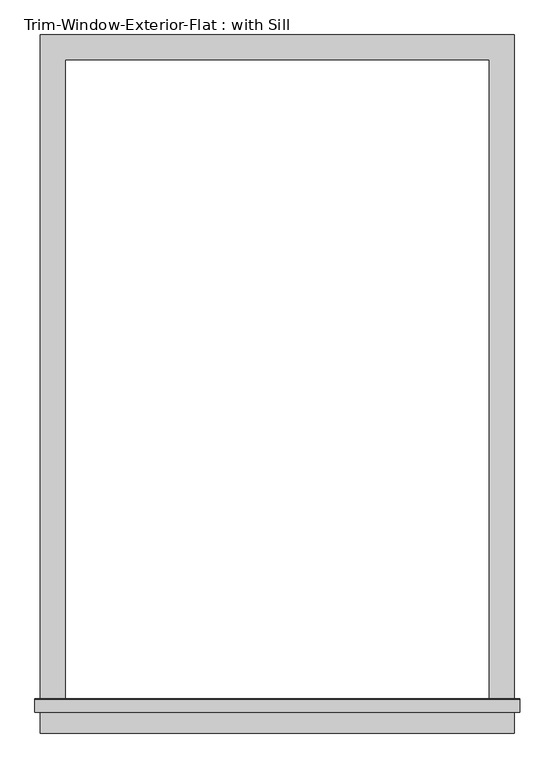
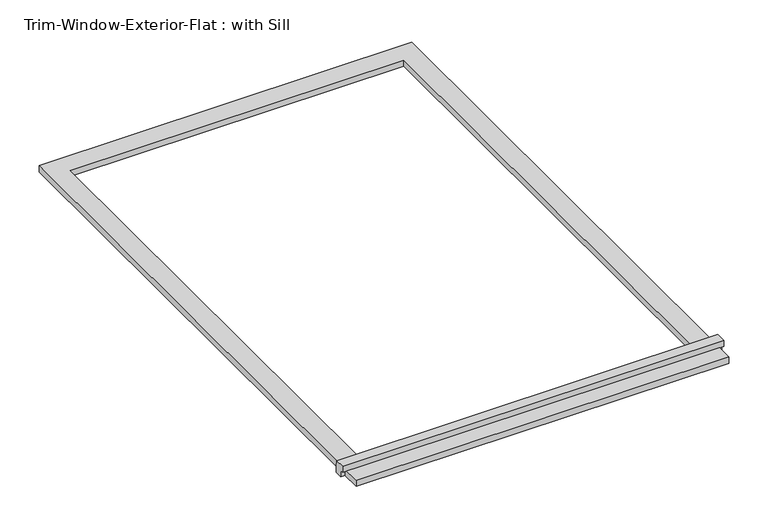
"""IFC4 building model written with IfcOpenShell, lengths in millimetres: proxy geometry, Trim-Window-Exterior-Flat : with Sill."""

import ifcopenshell
import ifcopenshell.guid

model = None  # the IFC model being written
_history = None  # IfcOwnerHistory: only IFC2X3 demands one
_inside = {}  # id of a spatial element -> (the spatial element, [elements in it])
_under = {}  # id of a project, library or spatial element -> (it, [spatial elements below it])
_declared = {}  # id of a project -> (the project, [libraries it declares])
_typed = {}  # id of a type object -> (the type object, [elements of that type])
_made_of = {}  # id of a material, layer set ... -> (it, [elements and type objects made of it])


def new_model(schema):
    """Start an empty IFC model of exactly this schema.

    Asked for "IFC4X3", IfcOpenShell would pick the latest addendum, in which some entities
    have other attributes; the version numbers below select the first issue.
    IFC2X3 requires an IfcOwnerHistory on every rooted entity: one is made here for all.
    """
    global model, _history
    if schema == "IFC4X3":
        model = ifcopenshell.file(schema_version=(4, 3, 0, 0))
    else:
        model = ifcopenshell.file(schema=schema)
    _inside.clear()
    _under.clear()
    _declared.clear()
    _typed.clear()
    _made_of.clear()
    _history = None
    if model.schema == "IFC2X3":
        org = make("IfcOrganization", Name="unknown")
        user = make(
            "IfcPersonAndOrganization",
            ThePerson=make("IfcPerson", FamilyName="unknown"),
            TheOrganization=org,
        )
        app = make(
            "IfcApplication",
            ApplicationDeveloper=org,
            Version="unknown",
            ApplicationFullName="unknown",
            ApplicationIdentifier="unknown",
        )
        _history = make(
            "IfcOwnerHistory",
            OwningUser=user,
            OwningApplication=app,
            ChangeAction="ADDED",
            CreationDate=0,
        )
    return model


def make(cls, **values):
    """One entity of the class cls with the attributes given. An attribute that is None is left unset."""
    return model.create_entity(
        cls, **{name: value for name, value in values.items() if value is not None}
    )


def rooted(cls, **values):
    """An entity with a GlobalId (a new one), such as an element, a storey or a relation."""
    return make(cls, GlobalId=ifcopenshell.guid.new(), OwnerHistory=_history, **values)


def si_unit(unit_type, name, prefix=None):
    """IfcSIUnit, for example si_unit("LENGTHUNIT", "METRE", prefix="MILLI")."""
    return make("IfcSIUnit", UnitType=unit_type, Prefix=prefix, Name=name)


def assignment(units):
    """IfcUnitAssignment: the units of a project."""
    return None if units is None else make("IfcUnitAssignment", Units=units)


def point(xyz):
    """IfcCartesianPoint."""
    return None if xyz is None else make("IfcCartesianPoint", Coordinates=xyz)


def direction(xyz):
    """IfcDirection."""
    return None if xyz is None else make("IfcDirection", DirectionRatios=xyz)


def frame(location, z_axis=None, x_axis=None):
    """IfcAxis2Placement3D, a coordinate frame: its origin and axes. An axis left out is left unset."""
    return make(
        "IfcAxis2Placement3D",
        Location=point(location),
        Axis=direction(z_axis),
        RefDirection=direction(x_axis),
    )


def origin():
    """The frame at (0, 0, 0) with its axes left unset."""
    return frame((0.0, 0.0, 0.0))


def origin_with_axes():
    """The frame at (0, 0, 0) with the z axis (0, 0, 1) and the x axis (1, 0, 0) written out."""
    return frame((0.0, 0.0, 0.0), z_axis=(0.0, 0.0, 1.0), x_axis=(1.0, 0.0, 0.0))


def place(relative_to, where):
    """IfcLocalPlacement: puts the frame where relative to a parent placement (None: the world)."""
    return make(
        "IfcLocalPlacement", PlacementRelTo=relative_to, RelativePlacement=where
    )


def context(
    kind, dimensions, precision=None, world=None, true_north=None, identifier=None
):
    """IfcGeometricRepresentationContext, for example the 3D "Model" context."""
    return make(
        "IfcGeometricRepresentationContext",
        ContextIdentifier=identifier,
        ContextType=kind,
        CoordinateSpaceDimension=dimensions,
        Precision=precision,
        WorldCoordinateSystem=world,
        TrueNorth=true_north,
    )


def project(units=None, contexts=None):
    """IfcProject with its units and contexts."""
    return rooted(
        "IfcProject",
        Name="project",
        RepresentationContexts=contexts,
        UnitsInContext=assignment(units),
    )


def spatial(cls, under=None, at=None, **own):
    """A site, building, storey or space (cls), placed at a placement, below another one or the project."""
    s = rooted(cls, ObjectPlacement=at, **own)
    if under is not None:
        _under.setdefault(under.id(), (under, []))[1].append(s)
    return s


def polyline(points):
    """IfcPolyline through the points."""
    return make("IfcPolyline", Points=[point(p) for p in points])


def outline(outer, holes=None, kind="AREA"):
    """IfcArbitraryClosedProfileDef: a profile drawn as a closed curve; with holes, ...WithVoids."""
    if holes is None:
        return make("IfcArbitraryClosedProfileDef", ProfileType=kind, OuterCurve=outer)
    return make(
        "IfcArbitraryProfileDefWithVoids",
        ProfileType=kind,
        OuterCurve=outer,
        InnerCurves=holes,
    )


def extrude(swept, where, along, depth):
    """IfcExtrudedAreaSolid: the profile swept, set in the frame where, extruded along a direction by depth."""
    return make(
        "IfcExtrudedAreaSolid",
        SweptArea=swept,
        Position=where,
        ExtrudedDirection=direction(along),
        Depth=depth,
    )


def shape(context_of_items, identifier, shape_type, items):
    """IfcShapeRepresentation: the items that make up one representation, for example the "Body"."""
    return make(
        "IfcShapeRepresentation",
        ContextOfItems=context_of_items,
        RepresentationIdentifier=identifier,
        RepresentationType=shape_type,
        Items=items,
    )


def source(mapping_origin, context_of_items, identifier, shape_type, items):
    """IfcRepresentationMap: a shape defined once, which mapped items show again and again."""
    return make(
        "IfcRepresentationMap",
        MappingOrigin=mapping_origin,
        MappedRepresentation=shape(context_of_items, identifier, shape_type, items),
    )


def transform(
    local_origin,
    x_axis=None,
    y_axis=None,
    z_axis=None,
    scale=None,
    scale2=None,
    scale3=None,
    uniform=True,
):
    """IfcCartesianTransformationOperator3D, or its non-uniform kind. x_axis, y_axis, z_axis: its Axis1, 2, 3."""
    if uniform:
        return make(
            "IfcCartesianTransformationOperator3D",
            Axis1=direction(x_axis),
            Axis2=direction(y_axis),
            LocalOrigin=point(local_origin),
            Scale=scale,
            Axis3=direction(z_axis),
        )
    return make(
        "IfcCartesianTransformationOperator3DnonUniform",
        Axis1=direction(x_axis),
        Axis2=direction(y_axis),
        LocalOrigin=point(local_origin),
        Scale=scale,
        Axis3=direction(z_axis),
        Scale2=scale2,
        Scale3=scale3,
    )


def mapped(mapping_source, mapping_target):
    """IfcMappedItem: shows the shape of a source again, moved by a transform."""
    return make(
        "IfcMappedItem", MappingSource=mapping_source, MappingTarget=mapping_target
    )


def made_of(thing, what):
    """Note that an element or type object is made of a material, layer set ...; save() writes the relation."""
    if what is not None:
        _made_of.setdefault(what.id(), (what, []))[1].append(thing)
    return thing


def element(
    cls,
    number,
    at=None,
    inside=None,
    cuts=None,
    type_object=None,
    material=None,
    context=None,
    identifier="Body",
    shape_type=None,
    held_by="IfcProductDefinitionShape",
    body=None,
    shapes=None,
    **own,
):
    """One element of the class cls, such as IfcWall. Its Tag is "e" and its number.

    at: its placement. inside: the storey or other place that contains it. cuts: it is an
    opening in that element (IfcRelVoidsElement). A single representation is given by context,
    identifier, shape_type and body (its items); several are given by shapes. held_by: the class
    of the entity that holds the representations. save() writes the other relations.
    """
    e = rooted(cls, Tag="e%d" % number, ObjectPlacement=at, **own)
    if body is not None:
        shapes = [shape(context, identifier, shape_type, body)]
    if shapes is not None:
        e.Representation = make(held_by, Representations=shapes)
    if inside is not None:
        _inside.setdefault(inside.id(), (inside, []))[1].append(e)
    if cuts is not None:
        rooted(
            "IfcRelVoidsElement", RelatingBuildingElement=cuts, RelatedOpeningElement=e
        )
    if type_object is not None:
        _typed.setdefault(type_object.id(), (type_object, []))[1].append(e)
    return made_of(e, material)


def aggregate(whole, parts):
    """IfcRelAggregates: a whole, such as a stair, and the parts it consists of."""
    return rooted("IfcRelAggregates", RelatingObject=whole, RelatedObjects=parts)


def save(model, path):
    """Write the relations noted so far, then the file.

    IfcRelAggregates (storeys below a building ...), IfcRelContainedInSpatialStructure (elements
    in a storey), IfcRelDefinesByType, IfcRelAssociatesMaterial and IfcRelDeclares: one each for
    every whole, place, type object, material and project.
    """
    for whole, parts in _under.values():
        aggregate(whole, parts)
    for where, things in _inside.values():
        rooted(
            "IfcRelContainedInSpatialStructure",
            RelatedElements=things,
            RelatingStructure=where,
        )
    for kind, things in _typed.values():
        rooted("IfcRelDefinesByType", RelatedObjects=things, RelatingType=kind)
    for what, things in _made_of.values():
        rooted("IfcRelAssociatesMaterial", RelatedObjects=things, RelatingMaterial=what)
    for by, libraries in _declared.values():
        rooted("IfcRelDeclares", RelatingContext=by, RelatedDefinitions=libraries)
    model.write(path)


def trim_window_exterior_flat_with_sill_6766514a(model_context):
    return source(origin(), model_context, "Body", "SweptSolid", [
        extrude(outline(polyline([(546.1, -1495.3823709), (546.1, -1552.5323709), (-546.1, -1552.5323709), (-546.1, -1495.3823709), (546.1, -1495.3823709)])), origin_with_axes(), (0.0, 0.0, 1.0), 19.05),
        extrude(outline(polyline([(-1504.95, 38.1), (-1475.6580645, 38.1), (-1473.2, 19.05), (-1473.2, 0.0), (-1495.3823709, 0.0), (-1495.3823709, 19.05), (-1504.95, 19.05), (-1504.95, 38.1)])), frame((-558.8, 0.0, 0.0), z_axis=(1.0, 0.0, 0.0), x_axis=(0.0, 1.0, 0.0)), (0.0, 0.0, 1.0), 1117.6),
        extrude(outline(polyline([(-546.1, 57.15), (546.1, 57.15), (546.1, -1473.2), (488.95, -1473.2), (488.95, 0.0), (-488.95, 0.0), (-488.95, -1473.2), (-546.1, -1473.2), (-546.1, 57.15)])), origin_with_axes(), (0.0, 0.0, 1.0), 19.05),
    ])


if __name__ == "__main__":
    model = new_model("IFC4")
    model_context = context("Model", 3, world=origin())
    ifc_project = project(units=[si_unit("LENGTHUNIT", "METRE", prefix="MILLI")], contexts=[model_context])
    site = spatial("IfcSite", under=ifc_project)
    building = spatial("IfcBuilding", under=site)
    placement = place(None, origin())
    trim_window_exterior_flat_with_sill_shape = trim_window_exterior_flat_with_sill_6766514a(model_context)
    element("IfcBuildingElementProxy", 1, Name="Trim-Window-Exterior-Flat : with Sill", ObjectType="Trim-Window-Exterior-Flat : with Sill", at=placement, inside=building, context=model_context, shape_type="MappedRepresentation", body=[
        mapped(trim_window_exterior_flat_with_sill_shape, transform((0.0, 0.0, 0.0), x_axis=(1.0, 0.0, 0.0), y_axis=(0.0, 1.0, 0.0), z_axis=(0.0, 0.0, 1.0))),
    ])
    save(model, "model.ifc")

# Revit data of these elements
# Type "Trim-Window-Exterior-Flat : with Sill"
#   Trim Width = 0' - 2 1/4"
#   Trim Thickness_Picture Frame = 0' - 1 1/4"
#   Trim Thickness_with Sill = 0' - 0 3/4"
#   Sill Thickness = 0' - 1 1/4"
#   Opening Width [instance default] = 2' - 0"
#   Opening Height [instance default] = 3' - 0"
#   Default Elevation = 4' - 0"
#   Sill = yes
#   Picture Frame = no
#   Trim Material [instance default] = none
# Element 1 (IfcBuildingElementProxy, "Trim-Window-Exterior-Flat : with Sill")
#   Opening Width = 3' - 2 1/2"
#   Opening Height = 4' - 10"
#   Trim Material = Clad - White
#   Materials on its faces: "Clad - White"
# Materials
#   "Clad - White": class "Wood", colour RGB 242 242 238, transparency 0, Cost = 0
